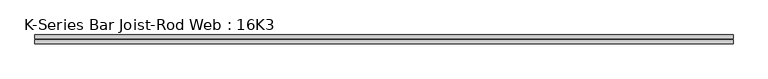
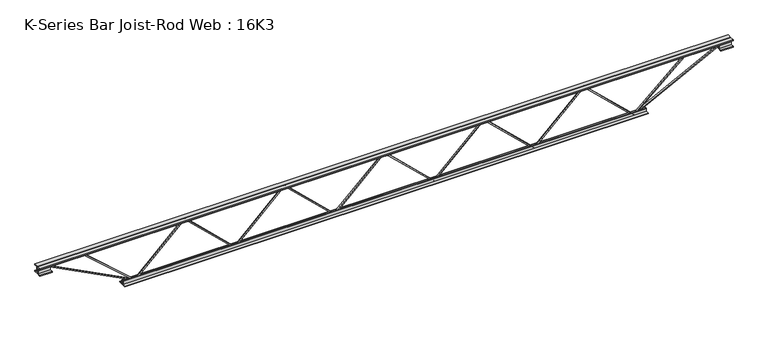
"""IFC4 building model written with IfcOpenShell, lengths in millimetres: beam geometry, K-Series Bar Joist-Rod Web : 16K3."""

from ifc_helpers import new_model, si_unit, frame, origin, place, context, project, spatial, polyline, outline, extrude, source, transform, mapped, element, save


def k_series_bar_joist_rod_web_16k3_999c0387(model_context):
    return source(origin(), model_context, "Body", "SweptSolid", [
        extrude(outline(polyline([(-192.0875, 418.1475), (-201.6125, 418.1475), (-201.6125, 423.2328103), (192.0875, 835.0303103), (192.0875, 837.5596897), (-201.6125, 1249.3571897), (-201.6125, 1254.4425), (-192.0875, 1254.4425), (-192.0875, 1253.1778103), (201.6125, 841.3803103), (201.6125, 831.2096897), (-192.0875, 419.4121897), (-192.0875, 418.1475)])), frame((0.0, -4.7625, 0.0), z_axis=(0.0, 1.0, 0.0), x_axis=(0.0, 0.0, 1.0)), (0.0, 0.0, 1.0), 9.525),
        extrude(outline(polyline([(-192.0875, -418.1475), (-201.6125, -418.1475), (-201.6125, -413.0621897), (192.0875, -1.2646897), (192.0875, 1.2646897), (-201.6125, 413.0621897), (-201.6125, 418.1475), (-192.0875, 418.1475), (-192.0875, 416.8828103), (201.6125, 5.0853103), (201.6125, -5.0853103), (-192.0875, -416.8828103), (-192.0875, -418.1475)])), frame((0.0, -4.7625, 0.0), z_axis=(0.0, 1.0, 0.0), x_axis=(0.0, 0.0, 1.0)), (0.0, 0.0, 1.0), 9.525),
        extrude(outline(polyline([(-192.0875, -1254.4425), (-201.6125, -1254.4425), (-201.6125, -1249.3571897), (192.0875, -837.5596897), (192.0875, -835.0303103), (-201.6125, -423.2328103), (-201.6125, -418.1475), (-192.0875, -418.1475), (-192.0875, -419.4121897), (201.6125, -831.2096897), (201.6125, -841.3803103), (-192.0875, -1253.1778103), (-192.0875, -1254.4425)])), frame((0.0, -4.7625, 0.0), z_axis=(0.0, 1.0, 0.0), x_axis=(0.0, 0.0, 1.0)), (0.0, 0.0, 1.0), 9.525),
        extrude(outline(polyline([(-192.0875, 1254.4425), (-201.6125, 1254.4425), (-201.6125, 1259.5278103), (192.0875, 1671.3253103), (192.0875, 1673.8546897), (-201.6125, 2085.6521897), (-201.6125, 2090.7375), (-192.0875, 2090.7375), (-192.0875, 2089.4728103), (201.6125, 1677.6753103), (201.6125, 1667.5046897), (-192.0875, 1255.7071897), (-192.0875, 1254.4425)])), frame((0.0, -4.7625, 0.0), z_axis=(0.0, 1.0, 0.0), x_axis=(0.0, 0.0, 1.0)), (0.0, 0.0, 1.0), 9.525),
        extrude(outline(polyline([(-192.0875, -2090.7375), (-201.6125, -2090.7375), (-201.6125, -2085.6521897), (192.0875, -1673.8546897), (192.0875, -1671.3253103), (-201.6125, -1259.5278103), (-201.6125, -1254.4425), (-192.0875, -1254.4425), (-192.0875, -1255.7071897), (201.6125, -1667.5046897), (201.6125, -1677.6753103), (-192.0875, -2089.4728103), (-192.0875, -2090.7375)])), frame((0.0, -4.7625, 0.0), z_axis=(0.0, 1.0, 0.0), x_axis=(0.0, 0.0, 1.0)), (0.0, 0.0, 1.0), 9.525),
        extrude(outline(polyline([(4.7625, 203.2), (36.5125, 203.2), (36.5125, 196.85), (11.1125, 196.85), (11.1125, 171.45), (4.7625, 171.45), (4.7625, 203.2)])), frame((-2903.5375, 0.0, 0.0), z_axis=(1.0, 0.0, 0.0), x_axis=(0.0, 1.0, 0.0)), (0.0, 0.0, 1.0), 5807.075),
        extrude(outline(polyline([(-4.7625, 203.2), (-4.7625, 171.45), (-11.1125, 171.45), (-11.1125, 196.85), (-36.5125, 196.85), (-36.5125, 203.2), (-4.7625, 203.2)])), frame((-2903.5375, 0.0, 0.0), z_axis=(1.0, 0.0, 0.0), x_axis=(0.0, 1.0, 0.0)), (0.0, 0.0, 1.0), 5807.075),
        extrude(outline(polyline([(-4.7625, 139.7), (-36.5125, 139.7), (-36.5125, 146.05), (-11.1125, 146.05), (-11.1125, 171.45), (-4.7625, 171.45), (-4.7625, 139.7)])), frame((-2903.5375, 0.0, 0.0), z_axis=(1.0, 0.0, 0.0), x_axis=(0.0, 1.0, 0.0)), (0.0, 0.0, 1.0), 101.6),
        extrude(outline(polyline([(36.5125, 139.7), (4.7625, 139.7), (4.7625, 171.45), (11.1125, 171.45), (11.1125, 146.05), (36.5125, 146.05), (36.5125, 139.7)])), frame((-2903.5375, 0.0, 0.0), z_axis=(1.0, 0.0, 0.0), x_axis=(0.0, 1.0, 0.0)), (0.0, 0.0, 1.0), 101.6),
        extrude(outline(polyline([(4.7625, 139.7), (4.7625, 171.45), (11.1125, 171.45), (11.1125, 146.05), (36.5125, 146.05), (36.5125, 139.7), (4.7625, 139.7)])), frame((2801.9375, 0.0, 0.0), z_axis=(1.0, 0.0, 0.0), x_axis=(0.0, 1.0, 0.0)), (0.0, 0.0, 1.0), 101.6),
        extrude(outline(polyline([(-4.7625, 139.7), (-36.5125, 139.7), (-36.5125, 146.05), (-11.1125, 146.05), (-11.1125, 171.45), (-4.7625, 171.45), (-4.7625, 139.7)])), frame((2801.9375, 0.0, 0.0), z_axis=(1.0, 0.0, 0.0), x_axis=(0.0, 1.0, 0.0)), (0.0, 0.0, 1.0), 101.6),
        extrude(outline(polyline([(4.7625, -203.2), (4.7625, -171.45), (11.1125, -171.45), (11.1125, -196.85), (36.5125, -196.85), (36.5125, -203.2), (4.7625, -203.2)])), frame((-2192.3375, 0.0, 0.0), z_axis=(1.0, 0.0, 0.0), x_axis=(0.0, 1.0, 0.0)), (0.0, 0.0, 1.0), 4384.675),
        extrude(outline(polyline([(-4.7625, -203.2), (-36.5125, -203.2), (-36.5125, -196.85), (-11.1125, -196.85), (-11.1125, -171.45), (-4.7625, -171.45), (-4.7625, -203.2)])), frame((-2192.3375, 0.0, 0.0), z_axis=(1.0, 0.0, 0.0), x_axis=(0.0, 1.0, 0.0)), (0.0, 0.0, 1.0), 4384.675),
        extrude(outline(polyline([(0.0, -9.525), (0.0, 0.0), (800.9059433, 0.0), (800.9059433, -9.525), (0.0, -9.525)])), frame((-2804.1275559, 4.7625, 167.2209266), z_axis=(0.45985424766113714, 0.0, 0.8879944092774513), x_axis=(0.8879944092774513, 0.0, -0.45985424766113714)), (0.0, 0.0, 1.0), 9.525),
        extrude(outline(polyline([(0.0, -9.525), (0.0, 0.0), (557.2182891, 0.0), (557.2182891, -9.525), (0.0, -9.525)])), frame((-2512.0328305, 4.7625, 167.8761269), z_axis=(0.6609617939242508, 0.0, 0.7504195539646047), x_axis=(0.7504195539646047, 0.0, -0.6609617939242508)), (0.0, 0.0, 1.0), 9.525),
        extrude(outline(polyline([(0.0, -9.525), (0.0, 0.0), (800.9059433, 0.0), (800.9059433, -9.525), (0.0, -9.525)])), frame((2804.1275559, -4.7625, 167.2209266), z_axis=(-0.4598542476611242, 0.0, 0.887994409277458), x_axis=(-0.887994409277458, 0.0, -0.4598542476611242)), (0.0, 0.0, 1.0), 9.525),
        extrude(outline(polyline([(0.0, -9.525), (0.0, 0.0), (557.2182891, 0.0), (557.2182891, -9.525), (0.0, -9.525)])), frame((2512.0328305, -4.7625, 167.8761269), z_axis=(-0.6609617939242457, 0.0, 0.7504195539646092), x_axis=(-0.7504195539646092, 0.0, -0.6609617939242457)), (0.0, 0.0, 1.0), 9.525),
    ])


if __name__ == "__main__":
    model = new_model("IFC4")
    model_context = context("Model", 3, world=origin())
    ifc_project = project(units=[si_unit("LENGTHUNIT", "METRE", prefix="MILLI")], contexts=[model_context])
    site = spatial("IfcSite", under=ifc_project)
    building = spatial("IfcBuilding", under=site)
    placement = place(None, origin())
    k_series_bar_joist_rod_web_16k3_shape = k_series_bar_joist_rod_web_16k3_999c0387(model_context)
    element("IfcBeam", 1, ObjectType="K-Series Bar Joist-Rod Web : 16K3", at=placement, inside=building, context=model_context, shape_type="MappedRepresentation", body=[
        mapped(k_series_bar_joist_rod_web_16k3_shape, transform((0.0, 0.0, 0.0), x_axis=(1.0, 0.0, 0.0), y_axis=(0.0, 1.0, 0.0), z_axis=(0.0, 0.0, 1.0))),
    ])
    save(model, "model.ifc")

# Revit data of these elements
# Type "K-Series Bar Joist-Rod Web : 16K3"
#   Assembly Code = "B1010350"
#   Wt = 6.3
#   Web Thickness = 0' - 0 3/8"
#   Start Offset [instance default] = 0' - 0"
#   Start Extension [instance default] = 0' - 0"
#   Seat Length = 0' - 4"
#   Seat Depth = 0' - 2 1/2"
#   PanelArrayLength [instance default] = 18' - 8"
#   Panel [instance default] = 2' - 8"
#   End Offset [instance default] = 0' - 0"
#   End Extension [instance default] = 0' - 0"
#   End Panel = 2' - 8"
#   Cord Leg = 0' - 1 1/4"
#   Chord Thickness = 0' - 0 1/4"
#   Length [instance default] = 24' - 0"
#   Depth = 1' - 4"
#   PanelArrayNum [instance default] = 7
#   Structural Material = none
# Element 1 (IfcBeam, "K-Series Bar Joist-Rod Web : 16K3")
#   PanelArrayLength = 13' - 8 5/8"
#   Panel = 2' - 8.925"
#   PanelArrayNum = 5
